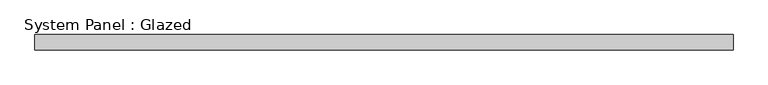
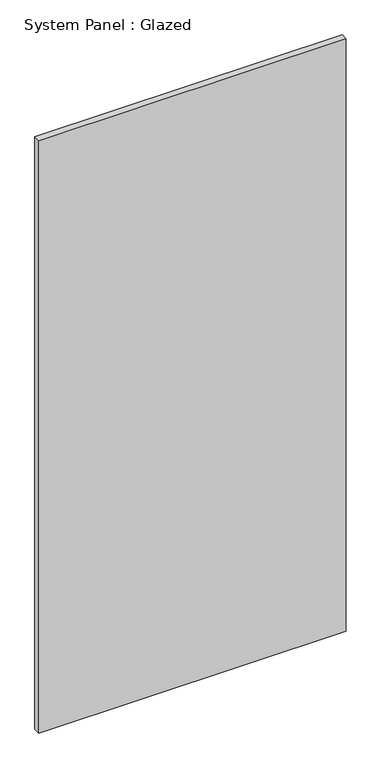
"""IFC4 building model written with IfcOpenShell, lengths in millimetres: plate geometry, System Panel : Glazed."""

from ifc_helpers import new_model, si_unit, origin, origin_with_axes, place, context, project, spatial, polyline, outline, extrude, source, transform, mapped, element, save


def system_panel_glazed_f2541063(model_context):
    return source(origin(), model_context, "Body", "SweptSolid", [
        extrude(outline(polyline([(583.1416667, 19.05), (-583.1416667, 19.05), (-583.1416667, 44.45), (583.1416667, 44.45), (583.1416667, 19.05)])), origin_with_axes(), (0.0, 0.0, 1.0), 2374.9),
    ])


if __name__ == "__main__":
    model = new_model("IFC4")
    model_context = context("Model", 3, world=origin())
    ifc_project = project(units=[si_unit("LENGTHUNIT", "METRE", prefix="MILLI")], contexts=[model_context])
    site = spatial("IfcSite", under=ifc_project)
    building = spatial("IfcBuilding", under=site)
    placement = place(None, origin())
    system_panel_glazed_shape = system_panel_glazed_f2541063(model_context)
    element("IfcPlate", 1, ObjectType="System Panel : Glazed", at=placement, inside=building, context=model_context, shape_type="MappedRepresentation", body=[
        mapped(system_panel_glazed_shape, transform((0.0, 0.0, 0.0), x_axis=(1.0, 0.0, 0.0), y_axis=(0.0, 1.0, 0.0), z_axis=(0.0, 0.0, 1.0))),
    ])
    save(model, "model.ifc")

# Revit data of these elements
# Element 1 (IfcPlate, "System Panel : Glazed")
#   Materials on its faces: "Glass"
# Materials
#   "Glass": class "Glass", colour RGB 218 227 224, transparency 0.85, Description = "Soda Lime Glass", Cost = 0
